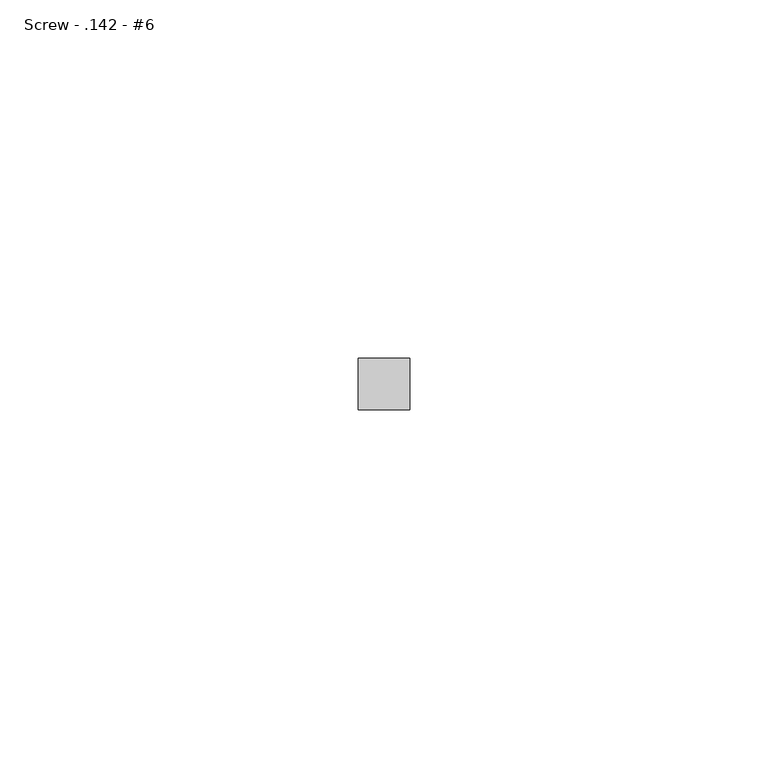
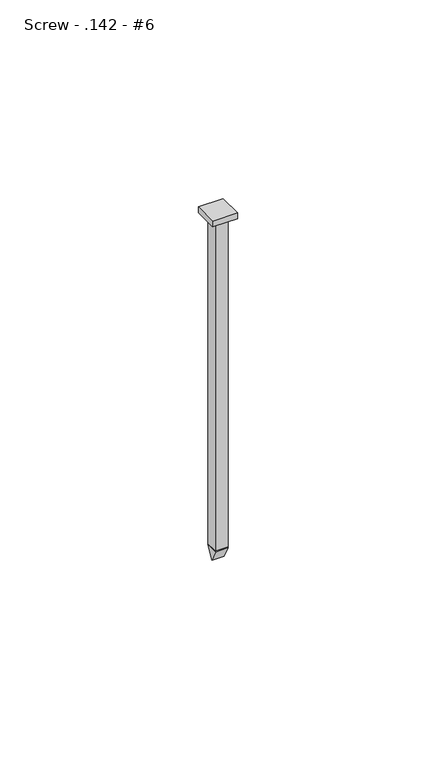
"""IFC4 building model written with IfcOpenShell, lengths in millimetres: fastener geometry, 060523 - W_P_C - Fastenings - Generic - SQUARE : Screw - .142 - #6."""

import ifcopenshell
import ifcopenshell.guid

model = None  # the IFC model being written
_history = None  # IfcOwnerHistory: only IFC2X3 demands one
_inside = {}  # id of a spatial element -> (the spatial element, [elements in it])
_under = {}  # id of a project, library or spatial element -> (it, [spatial elements below it])
_declared = {}  # id of a project -> (the project, [libraries it declares])
_typed = {}  # id of a type object -> (the type object, [elements of that type])
_made_of = {}  # id of a material, layer set ... -> (it, [elements and type objects made of it])


def new_model(schema):
    """Start an empty IFC model of exactly this schema.

    Asked for "IFC4X3", IfcOpenShell would pick the latest addendum, in which some entities
    have other attributes; the version numbers below select the first issue.
    IFC2X3 requires an IfcOwnerHistory on every rooted entity: one is made here for all.
    """
    global model, _history
    if schema == "IFC4X3":
        model = ifcopenshell.file(schema_version=(4, 3, 0, 0))
    else:
        model = ifcopenshell.file(schema=schema)
    _inside.clear()
    _under.clear()
    _declared.clear()
    _typed.clear()
    _made_of.clear()
    _history = None
    if model.schema == "IFC2X3":
        org = make("IfcOrganization", Name="unknown")
        user = make(
            "IfcPersonAndOrganization",
            ThePerson=make("IfcPerson", FamilyName="unknown"),
            TheOrganization=org,
        )
        app = make(
            "IfcApplication",
            ApplicationDeveloper=org,
            Version="unknown",
            ApplicationFullName="unknown",
            ApplicationIdentifier="unknown",
        )
        _history = make(
            "IfcOwnerHistory",
            OwningUser=user,
            OwningApplication=app,
            ChangeAction="ADDED",
            CreationDate=0,
        )
    return model


def make(cls, **values):
    """One entity of the class cls with the attributes given. An attribute that is None is left unset."""
    return model.create_entity(
        cls, **{name: value for name, value in values.items() if value is not None}
    )


def rooted(cls, **values):
    """An entity with a GlobalId (a new one), such as an element, a storey or a relation."""
    return make(cls, GlobalId=ifcopenshell.guid.new(), OwnerHistory=_history, **values)


def si_unit(unit_type, name, prefix=None):
    """IfcSIUnit, for example si_unit("LENGTHUNIT", "METRE", prefix="MILLI")."""
    return make("IfcSIUnit", UnitType=unit_type, Prefix=prefix, Name=name)


def assignment(units):
    """IfcUnitAssignment: the units of a project."""
    return None if units is None else make("IfcUnitAssignment", Units=units)


def point(xyz):
    """IfcCartesianPoint."""
    return None if xyz is None else make("IfcCartesianPoint", Coordinates=xyz)


def direction(xyz):
    """IfcDirection."""
    return None if xyz is None else make("IfcDirection", DirectionRatios=xyz)


def frame(location, z_axis=None, x_axis=None):
    """IfcAxis2Placement3D, a coordinate frame: its origin and axes. An axis left out is left unset."""
    return make(
        "IfcAxis2Placement3D",
        Location=point(location),
        Axis=direction(z_axis),
        RefDirection=direction(x_axis),
    )


def origin():
    """The frame at (0, 0, 0) with its axes left unset."""
    return frame((0.0, 0.0, 0.0))


def origin_with_axes():
    """The frame at (0, 0, 0) with the z axis (0, 0, 1) and the x axis (1, 0, 0) written out."""
    return frame((0.0, 0.0, 0.0), z_axis=(0.0, 0.0, 1.0), x_axis=(1.0, 0.0, 0.0))


def place(relative_to, where):
    """IfcLocalPlacement: puts the frame where relative to a parent placement (None: the world)."""
    return make(
        "IfcLocalPlacement", PlacementRelTo=relative_to, RelativePlacement=where
    )


def context(
    kind, dimensions, precision=None, world=None, true_north=None, identifier=None
):
    """IfcGeometricRepresentationContext, for example the 3D "Model" context."""
    return make(
        "IfcGeometricRepresentationContext",
        ContextIdentifier=identifier,
        ContextType=kind,
        CoordinateSpaceDimension=dimensions,
        Precision=precision,
        WorldCoordinateSystem=world,
        TrueNorth=true_north,
    )


def project(units=None, contexts=None):
    """IfcProject with its units and contexts."""
    return rooted(
        "IfcProject",
        Name="project",
        RepresentationContexts=contexts,
        UnitsInContext=assignment(units),
    )


def spatial(cls, under=None, at=None, **own):
    """A site, building, storey or space (cls), placed at a placement, below another one or the project."""
    s = rooted(cls, ObjectPlacement=at, **own)
    if under is not None:
        _under.setdefault(under.id(), (under, []))[1].append(s)
    return s


def polyline(points):
    """IfcPolyline through the points."""
    return make("IfcPolyline", Points=[point(p) for p in points])


def outline(outer, holes=None, kind="AREA"):
    """IfcArbitraryClosedProfileDef: a profile drawn as a closed curve; with holes, ...WithVoids."""
    if holes is None:
        return make("IfcArbitraryClosedProfileDef", ProfileType=kind, OuterCurve=outer)
    return make(
        "IfcArbitraryProfileDefWithVoids",
        ProfileType=kind,
        OuterCurve=outer,
        InnerCurves=holes,
    )


def extrude(swept, where, along, depth):
    """IfcExtrudedAreaSolid: the profile swept, set in the frame where, extruded along a direction by depth."""
    return make(
        "IfcExtrudedAreaSolid",
        SweptArea=swept,
        Position=where,
        ExtrudedDirection=direction(along),
        Depth=depth,
    )


def shape(context_of_items, identifier, shape_type, items):
    """IfcShapeRepresentation: the items that make up one representation, for example the "Body"."""
    return make(
        "IfcShapeRepresentation",
        ContextOfItems=context_of_items,
        RepresentationIdentifier=identifier,
        RepresentationType=shape_type,
        Items=items,
    )


def source(mapping_origin, context_of_items, identifier, shape_type, items):
    """IfcRepresentationMap: a shape defined once, which mapped items show again and again."""
    return make(
        "IfcRepresentationMap",
        MappingOrigin=mapping_origin,
        MappedRepresentation=shape(context_of_items, identifier, shape_type, items),
    )


def transform(
    local_origin,
    x_axis=None,
    y_axis=None,
    z_axis=None,
    scale=None,
    scale2=None,
    scale3=None,
    uniform=True,
):
    """IfcCartesianTransformationOperator3D, or its non-uniform kind. x_axis, y_axis, z_axis: its Axis1, 2, 3."""
    if uniform:
        return make(
            "IfcCartesianTransformationOperator3D",
            Axis1=direction(x_axis),
            Axis2=direction(y_axis),
            LocalOrigin=point(local_origin),
            Scale=scale,
            Axis3=direction(z_axis),
        )
    return make(
        "IfcCartesianTransformationOperator3DnonUniform",
        Axis1=direction(x_axis),
        Axis2=direction(y_axis),
        LocalOrigin=point(local_origin),
        Scale=scale,
        Axis3=direction(z_axis),
        Scale2=scale2,
        Scale3=scale3,
    )


def mapped(mapping_source, mapping_target):
    """IfcMappedItem: shows the shape of a source again, moved by a transform."""
    return make(
        "IfcMappedItem", MappingSource=mapping_source, MappingTarget=mapping_target
    )


def made_of(thing, what):
    """Note that an element or type object is made of a material, layer set ...; save() writes the relation."""
    if what is not None:
        _made_of.setdefault(what.id(), (what, []))[1].append(thing)
    return thing


def element(
    cls,
    number,
    at=None,
    inside=None,
    cuts=None,
    type_object=None,
    material=None,
    context=None,
    identifier="Body",
    shape_type=None,
    held_by="IfcProductDefinitionShape",
    body=None,
    shapes=None,
    **own,
):
    """One element of the class cls, such as IfcWall. Its Tag is "e" and its number.

    at: its placement. inside: the storey or other place that contains it. cuts: it is an
    opening in that element (IfcRelVoidsElement). A single representation is given by context,
    identifier, shape_type and body (its items); several are given by shapes. held_by: the class
    of the entity that holds the representations. save() writes the other relations.
    """
    e = rooted(cls, Tag="e%d" % number, ObjectPlacement=at, **own)
    if body is not None:
        shapes = [shape(context, identifier, shape_type, body)]
    if shapes is not None:
        e.Representation = make(held_by, Representations=shapes)
    if inside is not None:
        _inside.setdefault(inside.id(), (inside, []))[1].append(e)
    if cuts is not None:
        rooted(
            "IfcRelVoidsElement", RelatingBuildingElement=cuts, RelatedOpeningElement=e
        )
    if type_object is not None:
        _typed.setdefault(type_object.id(), (type_object, []))[1].append(e)
    return made_of(e, material)


def aggregate(whole, parts):
    """IfcRelAggregates: a whole, such as a stair, and the parts it consists of."""
    return rooted("IfcRelAggregates", RelatingObject=whole, RelatedObjects=parts)


def save(model, path):
    """Write the relations noted so far, then the file.

    IfcRelAggregates (storeys below a building ...), IfcRelContainedInSpatialStructure (elements
    in a storey), IfcRelDefinesByType, IfcRelAssociatesMaterial and IfcRelDeclares: one each for
    every whole, place, type object, material and project.
    """
    for whole, parts in _under.values():
        aggregate(whole, parts)
    for where, things in _inside.values():
        rooted(
            "IfcRelContainedInSpatialStructure",
            RelatedElements=things,
            RelatingStructure=where,
        )
    for kind, things in _typed.values():
        rooted("IfcRelDefinesByType", RelatedObjects=things, RelatingType=kind)
    for what, things in _made_of.values():
        rooted("IfcRelAssociatesMaterial", RelatedObjects=things, RelatingMaterial=what)
    for by, libraries in _declared.values():
        rooted("IfcRelDeclares", RelatingContext=by, RelatedDefinitions=libraries)
    model.write(path)


def screw_142_6_19bc7189(model_context):
    return source(origin(), model_context, "Body", "SweptSolid", [
        extrude(outline(polyline([(0.0, -105.2068), (-1.8034, -101.6), (1.8034, -101.6), (0.0, -105.2068)])), frame((-1.8034, 0.0, 0.0), z_axis=(1.0, 0.0, 0.0), x_axis=(0.0, 1.0, 0.0)), (0.0, 0.0, 1.0), 3.6068),
        extrude(outline(polyline([(-3.6068, -3.6068), (-3.6068, 3.6068), (3.6068, 3.6068), (3.6068, -3.6068), (-3.6068, -3.6068)])), origin_with_axes(), (0.0, 0.0, 1.0), 1.8034),
        extrude(outline(polyline([(-1.8034, 1.8034), (1.8034, 1.8034), (1.8034, -1.8034), (-1.8034, -1.8034), (-1.8034, 1.8034)])), frame((0.0, 0.0, -101.6), z_axis=(0.0, 0.0, 1.0), x_axis=(1.0, 0.0, 0.0)), (0.0, 0.0, 1.0), 101.6),
    ])


if __name__ == "__main__":
    model = new_model("IFC4")
    model_context = context("Model", 3, world=origin())
    ifc_project = project(units=[si_unit("LENGTHUNIT", "METRE", prefix="MILLI")], contexts=[model_context])
    site = spatial("IfcSite", under=ifc_project)
    building = spatial("IfcBuilding", under=site)
    placement = place(None, origin())
    screw_142_6_shape = screw_142_6_19bc7189(model_context)
    element("IfcFastener", 1, ObjectType="060523 - W_P_C - Fastenings - Generic - SQUARE : Screw - .142 - #6", at=placement, inside=building, context=model_context, shape_type="MappedRepresentation", body=[
        mapped(screw_142_6_shape, transform((0.0, 0.0, 0.0), x_axis=(1.0, 0.0, 0.0), y_axis=(0.0, 1.0, 0.0), z_axis=(0.0, 0.0, 1.0))),
    ])
    save(model, "model.ifc")

# Revit data of these elements
# Type "060523 - W_P_C - Fastenings - Generic - SQUARE : Screw - .142 - #6"
#   Washer_Thickness = 0' - 0.00333"
#   Washer Radius = 0' - 0.081"
#   Washer Offset - Head = 0' - 0"
#   Washer Offset = 0' - 0"
#   Thickness_of_Substrate [instance default] = 0' - 1"
#   Side = 0' - 0 37/64"
#   Radius = 0' - 0.071"
#   Length [instance default] = 0' - 4"
#   Head Size = 0' - 1"
#   Head Radius = 0' - 0 1/2"
#   Head Height = 0' - 0.01"
#   Double Diameter = 0' - 0.284"
#   Diameter = 0' - 0.142"
#   Default Elevation = 4' - 0"
#   Washer_Nut_Visibility = no
#   Washer_Head_Visibility = no
#   Round_Head_Visibility = yes
#   Point Visibility = yes
#   Nut_Visibility = no
#   Hex_Head_Visiblilty = no
#   Washer Material = none
#   Bolt Material (Size) = AT SILL - FASTENER AT 24" O.C.
# Materials
#   "AT SILL - FASTENER AT 24\" O.C.": class "Generic", colour RGB 120 120 120, transparency 0, Cost = 0
